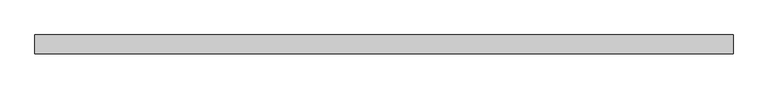
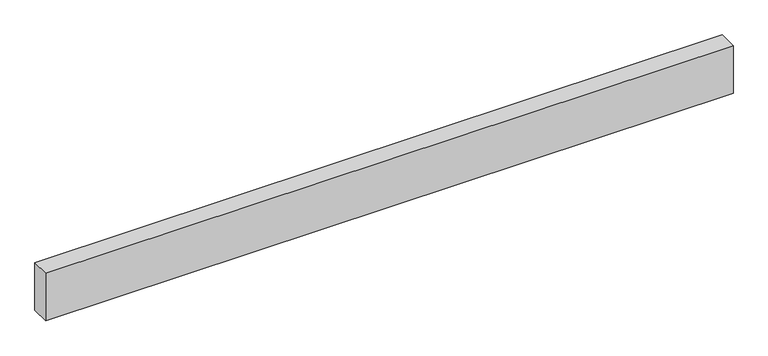
"""IFC4 building model written with IfcOpenShell, lengths in millimetres: beam geometry, NLRS_28_SF_LIB_houten balk-MMBW-SRP_gen_rsf : houten balk_gen__bxh 58x156."""

from ifc_helpers import new_model, si_unit, frame, origin, place, context, project, spatial, polyline, outline, extrude, source, transform, mapped, element, save


def beam_e7c6e874(model_context):
    return source(origin(), model_context, "Body", "SweptSolid", [
        extrude(outline(polyline([(-1067.0, -29.0), (-1067.0, 29.0), (1067.0, 29.0), (1067.0, -29.0), (-1067.0, -29.0)])), frame((0.0, 0.0, -78.0), z_axis=(0.0, 0.0, 1.0), x_axis=(1.0, 0.0, 0.0)), (0.0, 0.0, 1.0), 156.0),
    ])


if __name__ == "__main__":
    model = new_model("IFC4")
    model_context = context("Model", 3, world=origin())
    ifc_project = project(units=[si_unit("LENGTHUNIT", "METRE", prefix="MILLI")], contexts=[model_context])
    site = spatial("IfcSite", under=ifc_project)
    building = spatial("IfcBuilding", under=site)
    placement = place(None, origin())
    beam_shape = beam_e7c6e874(model_context)
    element("IfcBeam", 1, ObjectType="NLRS_28_SF_LIB_houten balk-MMBW-SRP_gen_rsf : houten balk_gen__bxh 58x156", at=placement, inside=building, context=model_context, shape_type="MappedRepresentation", body=[
        mapped(beam_shape, transform((0.0, 0.0, 0.0), x_axis=(1.0, 0.0, 0.0), y_axis=(0.0, 1.0, 0.0), z_axis=(0.0, 0.0, 1.0))),
    ])
    save(model, "model.ifc")

# Revit data of these elements
# Type "NLRS_28_SF_LIB_houten balk-MMBW-SRP_gen_rsf : houten balk_gen__bxh 58x156"
#   Type IfcGUID = "07M7mRoiH1CR8m_RSKIvXg"
#   IfcExportAs = "IfcBeamType"
#   Type Comments = "58x156"
#   Model = " "
#   Manufacturer = " "
#   Fire Rating = " "
#   Description = "houten balk 58x156"
#   Assembly Code = "28.11"
#   NLRS_C_lengte [instance default] = 3000 mm
#   NLRS_C_hoogte = 156 mm
#   NLRS_C_breedte = 58 mm
#   Length [instance default] = 3000 mm
#   Structural Material = NLRS_i2_hout naaldhout vuren_gen_rsf
#   Keynote = ""
# Element 1 (IfcBeam, "NLRS_28_SF_LIB_houten balk-MMBW-SRP_gen_rsf : houten balk_gen__bxh 58x156")
#   NLRS_C_lengte = 2250 mm
#   Materials on its faces: "NLRS_i2_hout naaldhout vuren_gen_rsf"
# Materials
#   "NLRS_i2_hout naaldhout vuren_gen_rsf": class "I - Hout", colour RGB 234 199 147, transparency 0, Keynote = "i2", Manufacturer = "Revit Standards Foundation", URL = "www.revitstandards.org", Description = "hout vuren", Cost = 0
